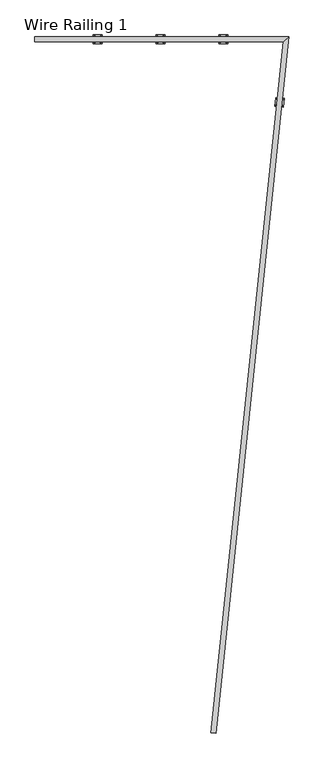
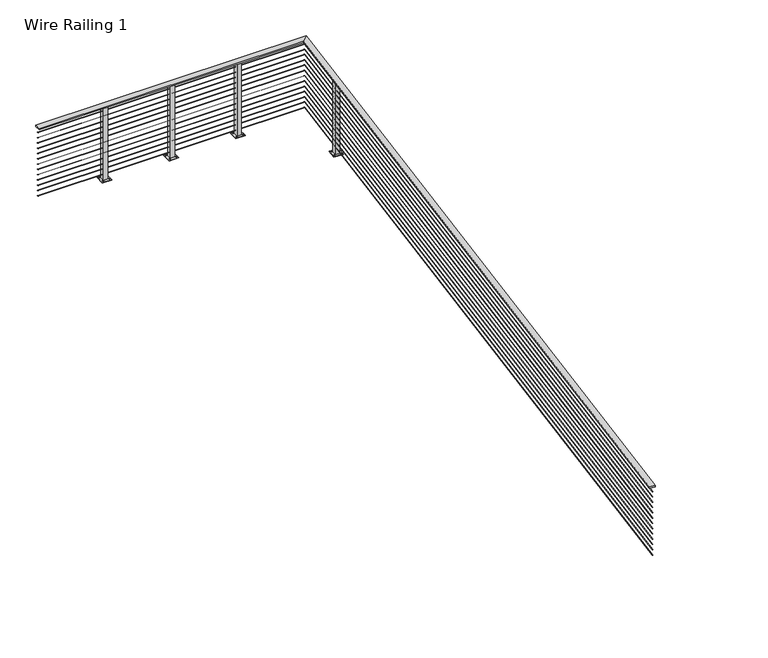
"""IFC4 building model written with IfcOpenShell, lengths in millimetres: railing geometry, Wire Railing 1."""

from ifc_helpers import new_model, si_unit, point, frame, frame_2d, origin, place, context, project, spatial, polyline, circle_curve, ellipse_curve, trimmed, segment, composite_curve, outline, extrude, faceted_brep, source, transform, mapped, element, save
from ifc_brep_helpers import plane_surface, cylinder_surface, advanced_brep


def wire_railing_1_df395d71(model_context):
    return source(origin(), model_context, "Body", "SolidModel", [
        faceted_brep([(31684.2784681, 40829.2481612, 270319.5), (31684.2784681, 40905.4481612, 270319.5), (31684.2784681, 40905.4481612, 270300.45), (31684.2784681, 40829.2481612, 270300.45), (35285.6983833, 40829.2481612, 270300.45), (35285.6983833, 40829.2481612, 270319.5), (35370.327057, 40905.4481612, 270300.45), (35370.327057, 40905.4481612, 270319.5), (34234.7001024, 30829.6674754, 270319.5), (34234.7001024, 30829.6674754, 270300.45), (34310.4826708, 30821.7024065, 270300.45), (34310.4826708, 30821.7024065, 270319.5)], [[[0, 1, 2, 3]], [[4, 5, 0, 3]], [[6, 4, 3, 2]], [[7, 6, 2, 1]], [[5, 7, 1, 0]], [[8, 9, 10, 11]], [[9, 8, 5, 4]], [[10, 9, 4, 6]], [[11, 10, 6, 7]], [[8, 11, 7, 5]]]),
        advanced_brep(
        [(31684.2784681, 40869.7294112, 270240.91875), (31684.2784681, 40864.9669112, 270240.91875), (35325.3680741, 40864.9669112, 270240.91875), (35330.6573662, 40869.7294112, 270240.91875), (34274.9595918, 30825.4360325, 270240.91875), (34270.2231813, 30825.9338493, 270240.91875)],
        [
            (0, 1, circle_curve(frame((31684.2784681, 40867.3481612, 270240.91875), z_axis=(-1.0, 0.0, 0.0), x_axis=(0.0, -1.0, 0.0)), 2.38125)),
            (1, 0, circle_curve(frame((31684.2784681, 40867.3481612, 270240.91875), z_axis=(-1.0, 0.0, 0.0), x_axis=(0.0, -1.0, 0.0)), 2.38125)),
            (2, 3, ellipse_curve(frame((35328.0127201, 40867.3481612, 270240.91875), z_axis=(-0.669130606358848, 0.7431448254774035, 0.0), x_axis=(0.7431448254774035, 0.6691306063588481, 0.0)), 3.5587223, 2.38125)),
            (3, 0),
            (1, 2),
            (3, 2, ellipse_curve(frame((35328.0127201, 40867.3481612, 270240.91875), z_axis=(-0.669130606358848, 0.7431448254774035, 0.0), x_axis=(0.7431448254774035, 0.6691306063588481, 0.0)), 3.5587223, 2.38125)),
            (4, 5, circle_curve(frame((34272.5913866, 30825.6849409, 270240.91875), z_axis=(-0.10452846326767264, -0.9945218953682714, 0.0), x_axis=(-0.9945218953682714, 0.10452846326767264, 0.0)), 2.38125)),
            (5, 4, circle_curve(frame((34272.5913866, 30825.6849409, 270240.91875), z_axis=(-0.10452846326767264, -0.9945218953682714, 0.0), x_axis=(-0.9945218953682714, 0.10452846326767264, 0.0)), 2.38125)),
            (4, 3),
            (2, 5),
        ],
        [
            plane_surface(frame((31684.2784681, 40867.3481612, 270243.3), z_axis=(-1.0, 0.0, 0.0), x_axis=(0.0, -1.0, 0.0))),
            cylinder_surface(frame((35328.0127201, 40867.3481612, 270240.91875), z_axis=(1.0, 0.0, 0.0), x_axis=(0.0, -1.0, 0.0)), 2.38125),
            plane_surface(frame((34272.5913866, 30825.6849409, 270243.3), z_axis=(-0.10452846326767265, -0.9945218953682714, 0.0), x_axis=(0.9945218953682714, -0.10452846326767265, 0.0))),
            cylinder_surface(frame((34272.5913866, 30825.6849409, 270240.91875), z_axis=(-0.10452846326767264, -0.9945218953682714, 0.0), x_axis=(-0.9945218953682714, 0.10452846326767264, 0.0)), 2.38125),
        ],
        [
            (0, [[1, 2]]),
            (1, [[3, 4, -2, 5]]),
            (1, [[6, -5, -1, -4]]),
            (2, [[7, 8]]),
            (3, [[-7, 9, -3, 10]]),
            (3, [[-8, -10, -6, -9]]),
        ],
    ),
        advanced_brep(
        [(31684.2784681, 40869.7294112, 270164.71875), (31684.2784681, 40864.9669112, 270164.71875), (35325.3680741, 40864.9669112, 270164.71875), (35330.6573662, 40869.7294112, 270164.71875), (34274.9595918, 30825.4360325, 270164.71875), (34270.2231813, 30825.9338493, 270164.71875)],
        [
            (0, 1, circle_curve(frame((31684.2784681, 40867.3481612, 270164.71875), z_axis=(-1.0, 0.0, 0.0), x_axis=(0.0, -1.0, 0.0)), 2.38125)),
            (1, 0, circle_curve(frame((31684.2784681, 40867.3481612, 270164.71875), z_axis=(-1.0, 0.0, 0.0), x_axis=(0.0, -1.0, 0.0)), 2.38125)),
            (2, 3, ellipse_curve(frame((35328.0127201, 40867.3481612, 270164.71875), z_axis=(-0.669130606358848, 0.7431448254774035, 0.0), x_axis=(0.7431448254774035, 0.6691306063588481, 0.0)), 3.5587223, 2.38125)),
            (3, 0),
            (1, 2),
            (3, 2, ellipse_curve(frame((35328.0127201, 40867.3481612, 270164.71875), z_axis=(-0.669130606358848, 0.7431448254774035, 0.0), x_axis=(0.7431448254774035, 0.6691306063588481, 0.0)), 3.5587223, 2.38125)),
            (4, 5, circle_curve(frame((34272.5913866, 30825.6849409, 270164.71875), z_axis=(-0.10452846326767264, -0.9945218953682714, 0.0), x_axis=(-0.9945218953682714, 0.10452846326767264, 0.0)), 2.38125)),
            (5, 4, circle_curve(frame((34272.5913866, 30825.6849409, 270164.71875), z_axis=(-0.10452846326767264, -0.9945218953682714, 0.0), x_axis=(-0.9945218953682714, 0.10452846326767264, 0.0)), 2.38125)),
            (4, 3),
            (2, 5),
        ],
        [
            plane_surface(frame((31684.2784681, 40867.3481612, 270167.1), z_axis=(-1.0, 0.0, 0.0), x_axis=(0.0, -1.0, 0.0))),
            cylinder_surface(frame((35328.0127201, 40867.3481612, 270164.71875), z_axis=(1.0, 0.0, 0.0), x_axis=(0.0, -1.0, 0.0)), 2.38125),
            plane_surface(frame((34272.5913866, 30825.6849409, 270167.1), z_axis=(-0.10452846326767265, -0.9945218953682714, 0.0), x_axis=(0.9945218953682714, -0.10452846326767265, 0.0))),
            cylinder_surface(frame((34272.5913866, 30825.6849409, 270164.71875), z_axis=(-0.10452846326767264, -0.9945218953682714, 0.0), x_axis=(-0.9945218953682714, 0.10452846326767264, 0.0)), 2.38125),
        ],
        [
            (0, [[1, 2]]),
            (1, [[3, 4, -2, 5]]),
            (1, [[6, -5, -1, -4]]),
            (2, [[7, 8]]),
            (3, [[-7, 9, -3, 10]]),
            (3, [[-8, -10, -6, -9]]),
        ],
    ),
        advanced_brep(
        [(31684.2784681, 40869.7294112, 270088.51875), (31684.2784681, 40864.9669112, 270088.51875), (35325.3680741, 40864.9669112, 270088.51875), (35330.6573662, 40869.7294112, 270088.51875), (34274.9595918, 30825.4360325, 270088.51875), (34270.2231813, 30825.9338493, 270088.51875)],
        [
            (0, 1, circle_curve(frame((31684.2784681, 40867.3481612, 270088.51875), z_axis=(-1.0, 0.0, 0.0), x_axis=(0.0, -1.0, 0.0)), 2.38125)),
            (1, 0, circle_curve(frame((31684.2784681, 40867.3481612, 270088.51875), z_axis=(-1.0, 0.0, 0.0), x_axis=(0.0, -1.0, 0.0)), 2.38125)),
            (2, 3, ellipse_curve(frame((35328.0127201, 40867.3481612, 270088.51875), z_axis=(-0.669130606358848, 0.7431448254774035, 0.0), x_axis=(0.7431448254774035, 0.6691306063588481, 0.0)), 3.5587223, 2.38125)),
            (3, 0),
            (1, 2),
            (3, 2, ellipse_curve(frame((35328.0127201, 40867.3481612, 270088.51875), z_axis=(-0.669130606358848, 0.7431448254774035, 0.0), x_axis=(0.7431448254774035, 0.6691306063588481, 0.0)), 3.5587223, 2.38125)),
            (4, 5, circle_curve(frame((34272.5913866, 30825.6849409, 270088.51875), z_axis=(-0.10452846326767264, -0.9945218953682714, 0.0), x_axis=(-0.9945218953682714, 0.10452846326767264, 0.0)), 2.38125)),
            (5, 4, circle_curve(frame((34272.5913866, 30825.6849409, 270088.51875), z_axis=(-0.10452846326767264, -0.9945218953682714, 0.0), x_axis=(-0.9945218953682714, 0.10452846326767264, 0.0)), 2.38125)),
            (4, 3),
            (2, 5),
        ],
        [
            plane_surface(frame((31684.2784681, 40867.3481612, 270090.9), z_axis=(-1.0, 0.0, 0.0), x_axis=(0.0, -1.0, 0.0))),
            cylinder_surface(frame((35328.0127201, 40867.3481612, 270088.51875), z_axis=(1.0, 0.0, 0.0), x_axis=(0.0, -1.0, 0.0)), 2.38125),
            plane_surface(frame((34272.5913866, 30825.6849409, 270090.9), z_axis=(-0.10452846326767265, -0.9945218953682714, 0.0), x_axis=(0.9945218953682714, -0.10452846326767265, 0.0))),
            cylinder_surface(frame((34272.5913866, 30825.6849409, 270088.51875), z_axis=(-0.10452846326767264, -0.9945218953682714, 0.0), x_axis=(-0.9945218953682714, 0.10452846326767264, 0.0)), 2.38125),
        ],
        [
            (0, [[1, 2]]),
            (1, [[3, 4, -2, 5]]),
            (1, [[6, -5, -1, -4]]),
            (2, [[7, 8]]),
            (3, [[-7, 9, -3, 10]]),
            (3, [[-8, -10, -6, -9]]),
        ],
    ),
        advanced_brep(
        [(31684.2784681, 40869.7294112, 270012.31875), (31684.2784681, 40864.9669112, 270012.31875), (35325.3680741, 40864.9669112, 270012.31875), (35330.6573662, 40869.7294112, 270012.31875), (34274.9595918, 30825.4360325, 270012.31875), (34270.2231813, 30825.9338493, 270012.31875)],
        [
            (0, 1, circle_curve(frame((31684.2784681, 40867.3481612, 270012.31875), z_axis=(-1.0, 0.0, 0.0), x_axis=(0.0, -1.0, 0.0)), 2.38125)),
            (1, 0, circle_curve(frame((31684.2784681, 40867.3481612, 270012.31875), z_axis=(-1.0, 0.0, 0.0), x_axis=(0.0, -1.0, 0.0)), 2.38125)),
            (2, 3, ellipse_curve(frame((35328.0127201, 40867.3481612, 270012.31875), z_axis=(-0.669130606358848, 0.7431448254774035, 0.0), x_axis=(0.7431448254774035, 0.6691306063588481, 0.0)), 3.5587223, 2.38125)),
            (3, 0),
            (1, 2),
            (3, 2, ellipse_curve(frame((35328.0127201, 40867.3481612, 270012.31875), z_axis=(-0.669130606358848, 0.7431448254774035, 0.0), x_axis=(0.7431448254774035, 0.6691306063588481, 0.0)), 3.5587223, 2.38125)),
            (4, 5, circle_curve(frame((34272.5913866, 30825.6849409, 270012.31875), z_axis=(-0.10452846326767264, -0.9945218953682714, 0.0), x_axis=(-0.9945218953682714, 0.10452846326767264, 0.0)), 2.38125)),
            (5, 4, circle_curve(frame((34272.5913866, 30825.6849409, 270012.31875), z_axis=(-0.10452846326767264, -0.9945218953682714, 0.0), x_axis=(-0.9945218953682714, 0.10452846326767264, 0.0)), 2.38125)),
            (4, 3),
            (2, 5),
        ],
        [
            plane_surface(frame((31684.2784681, 40867.3481612, 270014.7), z_axis=(-1.0, 0.0, 0.0), x_axis=(0.0, -1.0, 0.0))),
            cylinder_surface(frame((35328.0127201, 40867.3481612, 270012.31875), z_axis=(1.0, 0.0, 0.0), x_axis=(0.0, -1.0, 0.0)), 2.38125),
            plane_surface(frame((34272.5913866, 30825.6849409, 270014.7), z_axis=(-0.10452846326767265, -0.9945218953682714, 0.0), x_axis=(0.9945218953682714, -0.10452846326767265, 0.0))),
            cylinder_surface(frame((34272.5913866, 30825.6849409, 270012.31875), z_axis=(-0.10452846326767264, -0.9945218953682714, 0.0), x_axis=(-0.9945218953682714, 0.10452846326767264, 0.0)), 2.38125),
        ],
        [
            (0, [[1, 2]]),
            (1, [[3, 4, -2, 5]]),
            (1, [[6, -5, -1, -4]]),
            (2, [[7, 8]]),
            (3, [[-7, 9, -3, 10]]),
            (3, [[-8, -10, -6, -9]]),
        ],
    ),
        advanced_brep(
        [(31684.2784681, 40869.7294112, 269936.11875), (31684.2784681, 40864.9669112, 269936.11875), (35325.3680741, 40864.9669112, 269936.11875), (35330.6573662, 40869.7294112, 269936.11875), (34274.9595918, 30825.4360325, 269936.11875), (34270.2231813, 30825.9338493, 269936.11875)],
        [
            (0, 1, circle_curve(frame((31684.2784681, 40867.3481612, 269936.11875), z_axis=(-1.0, 0.0, 0.0), x_axis=(0.0, -1.0, 0.0)), 2.38125)),
            (1, 0, circle_curve(frame((31684.2784681, 40867.3481612, 269936.11875), z_axis=(-1.0, 0.0, 0.0), x_axis=(0.0, -1.0, 0.0)), 2.38125)),
            (2, 3, ellipse_curve(frame((35328.0127201, 40867.3481612, 269936.11875), z_axis=(-0.669130606358848, 0.7431448254774035, 0.0), x_axis=(0.7431448254774035, 0.6691306063588481, 0.0)), 3.5587223, 2.38125)),
            (3, 0),
            (1, 2),
            (3, 2, ellipse_curve(frame((35328.0127201, 40867.3481612, 269936.11875), z_axis=(-0.669130606358848, 0.7431448254774035, 0.0), x_axis=(0.7431448254774035, 0.6691306063588481, 0.0)), 3.5587223, 2.38125)),
            (4, 5, circle_curve(frame((34272.5913866, 30825.6849409, 269936.11875), z_axis=(-0.10452846326767264, -0.9945218953682714, 0.0), x_axis=(-0.9945218953682714, 0.10452846326767264, 0.0)), 2.38125)),
            (5, 4, circle_curve(frame((34272.5913866, 30825.6849409, 269936.11875), z_axis=(-0.10452846326767264, -0.9945218953682714, 0.0), x_axis=(-0.9945218953682714, 0.10452846326767264, 0.0)), 2.38125)),
            (4, 3),
            (2, 5),
        ],
        [
            plane_surface(frame((31684.2784681, 40867.3481612, 269938.5), z_axis=(-1.0, 0.0, 0.0), x_axis=(0.0, -1.0, 0.0))),
            cylinder_surface(frame((35328.0127201, 40867.3481612, 269936.11875), z_axis=(1.0, 0.0, 0.0), x_axis=(0.0, -1.0, 0.0)), 2.38125),
            plane_surface(frame((34272.5913866, 30825.6849409, 269938.5), z_axis=(-0.10452846326767265, -0.9945218953682714, 0.0), x_axis=(0.9945218953682714, -0.10452846326767265, 0.0))),
            cylinder_surface(frame((34272.5913866, 30825.6849409, 269936.11875), z_axis=(-0.10452846326767264, -0.9945218953682714, 0.0), x_axis=(-0.9945218953682714, 0.10452846326767264, 0.0)), 2.38125),
        ],
        [
            (0, [[1, 2]]),
            (1, [[3, 4, -2, 5]]),
            (1, [[6, -5, -1, -4]]),
            (2, [[7, 8]]),
            (3, [[-7, 9, -3, 10]]),
            (3, [[-8, -10, -6, -9]]),
        ],
    ),
        advanced_brep(
        [(31684.2784681, 40869.7294112, 269859.91875), (31684.2784681, 40864.9669112, 269859.91875), (35325.3680741, 40864.9669112, 269859.91875), (35330.6573662, 40869.7294112, 269859.91875), (34274.9595918, 30825.4360325, 269859.91875), (34270.2231813, 30825.9338493, 269859.91875)],
        [
            (0, 1, circle_curve(frame((31684.2784681, 40867.3481612, 269859.91875), z_axis=(-1.0, 0.0, 0.0), x_axis=(0.0, -1.0, 0.0)), 2.38125)),
            (1, 0, circle_curve(frame((31684.2784681, 40867.3481612, 269859.91875), z_axis=(-1.0, 0.0, 0.0), x_axis=(0.0, -1.0, 0.0)), 2.38125)),
            (2, 3, ellipse_curve(frame((35328.0127201, 40867.3481612, 269859.91875), z_axis=(-0.669130606358848, 0.7431448254774035, 0.0), x_axis=(0.7431448254774035, 0.6691306063588481, 0.0)), 3.5587223, 2.38125)),
            (3, 0),
            (1, 2),
            (3, 2, ellipse_curve(frame((35328.0127201, 40867.3481612, 269859.91875), z_axis=(-0.669130606358848, 0.7431448254774035, 0.0), x_axis=(0.7431448254774035, 0.6691306063588481, 0.0)), 3.5587223, 2.38125)),
            (4, 5, circle_curve(frame((34272.5913866, 30825.6849409, 269859.91875), z_axis=(-0.10452846326767264, -0.9945218953682714, 0.0), x_axis=(-0.9945218953682714, 0.10452846326767264, 0.0)), 2.38125)),
            (5, 4, circle_curve(frame((34272.5913866, 30825.6849409, 269859.91875), z_axis=(-0.10452846326767264, -0.9945218953682714, 0.0), x_axis=(-0.9945218953682714, 0.10452846326767264, 0.0)), 2.38125)),
            (4, 3),
            (2, 5),
        ],
        [
            plane_surface(frame((31684.2784681, 40867.3481612, 269862.3), z_axis=(-1.0, 0.0, 0.0), x_axis=(0.0, -1.0, 0.0))),
            cylinder_surface(frame((35328.0127201, 40867.3481612, 269859.91875), z_axis=(1.0, 0.0, 0.0), x_axis=(0.0, -1.0, 0.0)), 2.38125),
            plane_surface(frame((34272.5913866, 30825.6849409, 269862.3), z_axis=(-0.10452846326767265, -0.9945218953682714, 0.0), x_axis=(0.9945218953682714, -0.10452846326767265, 0.0))),
            cylinder_surface(frame((34272.5913866, 30825.6849409, 269859.91875), z_axis=(-0.10452846326767264, -0.9945218953682714, 0.0), x_axis=(-0.9945218953682714, 0.10452846326767264, 0.0)), 2.38125),
        ],
        [
            (0, [[1, 2]]),
            (1, [[3, 4, -2, 5]]),
            (1, [[6, -5, -1, -4]]),
            (2, [[7, 8]]),
            (3, [[-7, 9, -3, 10]]),
            (3, [[-8, -10, -6, -9]]),
        ],
    ),
        advanced_brep(
        [(31684.2784681, 40869.7294112, 269783.71875), (31684.2784681, 40864.9669112, 269783.71875), (35325.3680741, 40864.9669112, 269783.71875), (35330.6573662, 40869.7294112, 269783.71875), (34274.9595918, 30825.4360325, 269783.71875), (34270.2231813, 30825.9338493, 269783.71875)],
        [
            (0, 1, circle_curve(frame((31684.2784681, 40867.3481612, 269783.71875), z_axis=(-1.0, 0.0, 0.0), x_axis=(0.0, -1.0, 0.0)), 2.38125)),
            (1, 0, circle_curve(frame((31684.2784681, 40867.3481612, 269783.71875), z_axis=(-1.0, 0.0, 0.0), x_axis=(0.0, -1.0, 0.0)), 2.38125)),
            (2, 3, ellipse_curve(frame((35328.0127201, 40867.3481612, 269783.71875), z_axis=(-0.669130606358848, 0.7431448254774035, 0.0), x_axis=(0.7431448254774035, 0.6691306063588481, 0.0)), 3.5587223, 2.38125)),
            (3, 0),
            (1, 2),
            (3, 2, ellipse_curve(frame((35328.0127201, 40867.3481612, 269783.71875), z_axis=(-0.669130606358848, 0.7431448254774035, 0.0), x_axis=(0.7431448254774035, 0.6691306063588481, 0.0)), 3.5587223, 2.38125)),
            (4, 5, circle_curve(frame((34272.5913866, 30825.6849409, 269783.71875), z_axis=(-0.10452846326767264, -0.9945218953682714, 0.0), x_axis=(-0.9945218953682714, 0.10452846326767264, 0.0)), 2.38125)),
            (5, 4, circle_curve(frame((34272.5913866, 30825.6849409, 269783.71875), z_axis=(-0.10452846326767264, -0.9945218953682714, 0.0), x_axis=(-0.9945218953682714, 0.10452846326767264, 0.0)), 2.38125)),
            (4, 3),
            (2, 5),
        ],
        [
            plane_surface(frame((31684.2784681, 40867.3481612, 269786.1), z_axis=(-1.0, 0.0, 0.0), x_axis=(0.0, -1.0, 0.0))),
            cylinder_surface(frame((35328.0127201, 40867.3481612, 269783.71875), z_axis=(1.0, 0.0, 0.0), x_axis=(0.0, -1.0, 0.0)), 2.38125),
            plane_surface(frame((34272.5913866, 30825.6849409, 269786.1), z_axis=(-0.10452846326767265, -0.9945218953682714, 0.0), x_axis=(0.9945218953682714, -0.10452846326767265, 0.0))),
            cylinder_surface(frame((34272.5913866, 30825.6849409, 269783.71875), z_axis=(-0.10452846326767264, -0.9945218953682714, 0.0), x_axis=(-0.9945218953682714, 0.10452846326767264, 0.0)), 2.38125),
        ],
        [
            (0, [[1, 2]]),
            (1, [[3, 4, -2, 5]]),
            (1, [[6, -5, -1, -4]]),
            (2, [[7, 8]]),
            (3, [[-7, 9, -3, 10]]),
            (3, [[-8, -10, -6, -9]]),
        ],
    ),
        advanced_brep(
        [(31684.2784681, 40869.7294112, 269707.51875), (31684.2784681, 40864.9669112, 269707.51875), (35325.3680741, 40864.9669112, 269707.51875), (35330.6573662, 40869.7294112, 269707.51875), (34274.9595918, 30825.4360325, 269707.51875), (34270.2231813, 30825.9338493, 269707.51875)],
        [
            (0, 1, circle_curve(frame((31684.2784681, 40867.3481612, 269707.51875), z_axis=(-1.0, 0.0, 0.0), x_axis=(0.0, -1.0, 0.0)), 2.38125)),
            (1, 0, circle_curve(frame((31684.2784681, 40867.3481612, 269707.51875), z_axis=(-1.0, 0.0, 0.0), x_axis=(0.0, -1.0, 0.0)), 2.38125)),
            (2, 3, ellipse_curve(frame((35328.0127201, 40867.3481612, 269707.51875), z_axis=(-0.669130606358848, 0.7431448254774035, 0.0), x_axis=(0.7431448254774035, 0.6691306063588481, 0.0)), 3.5587223, 2.38125)),
            (3, 0),
            (1, 2),
            (3, 2, ellipse_curve(frame((35328.0127201, 40867.3481612, 269707.51875), z_axis=(-0.669130606358848, 0.7431448254774035, 0.0), x_axis=(0.7431448254774035, 0.6691306063588481, 0.0)), 3.5587223, 2.38125)),
            (4, 5, circle_curve(frame((34272.5913866, 30825.6849409, 269707.51875), z_axis=(-0.10452846326767264, -0.9945218953682714, 0.0), x_axis=(-0.9945218953682714, 0.10452846326767264, 0.0)), 2.38125)),
            (5, 4, circle_curve(frame((34272.5913866, 30825.6849409, 269707.51875), z_axis=(-0.10452846326767264, -0.9945218953682714, 0.0), x_axis=(-0.9945218953682714, 0.10452846326767264, 0.0)), 2.38125)),
            (4, 3),
            (2, 5),
        ],
        [
            plane_surface(frame((31684.2784681, 40867.3481612, 269709.9), z_axis=(-1.0, 0.0, 0.0), x_axis=(0.0, -1.0, 0.0))),
            cylinder_surface(frame((35328.0127201, 40867.3481612, 269707.51875), z_axis=(1.0, 0.0, 0.0), x_axis=(0.0, -1.0, 0.0)), 2.38125),
            plane_surface(frame((34272.5913866, 30825.6849409, 269709.9), z_axis=(-0.10452846326767265, -0.9945218953682714, 0.0), x_axis=(0.9945218953682714, -0.10452846326767265, 0.0))),
            cylinder_surface(frame((34272.5913866, 30825.6849409, 269707.51875), z_axis=(-0.10452846326767264, -0.9945218953682714, 0.0), x_axis=(-0.9945218953682714, 0.10452846326767264, 0.0)), 2.38125),
        ],
        [
            (0, [[1, 2]]),
            (1, [[3, 4, -2, 5]]),
            (1, [[6, -5, -1, -4]]),
            (2, [[7, 8]]),
            (3, [[-7, 9, -3, 10]]),
            (3, [[-8, -10, -6, -9]]),
        ],
    ),
        advanced_brep(
        [(31684.2784681, 40869.7294112, 269631.31875), (31684.2784681, 40864.9669112, 269631.31875), (35325.3680741, 40864.9669112, 269631.31875), (35330.6573662, 40869.7294112, 269631.31875), (34274.9595918, 30825.4360325, 269631.31875), (34270.2231813, 30825.9338493, 269631.31875)],
        [
            (0, 1, circle_curve(frame((31684.2784681, 40867.3481612, 269631.31875), z_axis=(-1.0, 0.0, 0.0), x_axis=(0.0, -1.0, 0.0)), 2.38125)),
            (1, 0, circle_curve(frame((31684.2784681, 40867.3481612, 269631.31875), z_axis=(-1.0, 0.0, 0.0), x_axis=(0.0, -1.0, 0.0)), 2.38125)),
            (2, 3, ellipse_curve(frame((35328.0127201, 40867.3481612, 269631.31875), z_axis=(-0.669130606358848, 0.7431448254774035, 0.0), x_axis=(0.7431448254774035, 0.6691306063588481, 0.0)), 3.5587223, 2.38125)),
            (3, 0),
            (1, 2),
            (3, 2, ellipse_curve(frame((35328.0127201, 40867.3481612, 269631.31875), z_axis=(-0.669130606358848, 0.7431448254774035, 0.0), x_axis=(0.7431448254774035, 0.6691306063588481, 0.0)), 3.5587223, 2.38125)),
            (4, 5, circle_curve(frame((34272.5913866, 30825.6849409, 269631.31875), z_axis=(-0.10452846326767264, -0.9945218953682714, 0.0), x_axis=(-0.9945218953682714, 0.10452846326767264, 0.0)), 2.38125)),
            (5, 4, circle_curve(frame((34272.5913866, 30825.6849409, 269631.31875), z_axis=(-0.10452846326767264, -0.9945218953682714, 0.0), x_axis=(-0.9945218953682714, 0.10452846326767264, 0.0)), 2.38125)),
            (4, 3),
            (2, 5),
        ],
        [
            plane_surface(frame((31684.2784681, 40867.3481612, 269633.7), z_axis=(-1.0, 0.0, 0.0), x_axis=(0.0, -1.0, 0.0))),
            cylinder_surface(frame((35328.0127201, 40867.3481612, 269631.31875), z_axis=(1.0, 0.0, 0.0), x_axis=(0.0, -1.0, 0.0)), 2.38125),
            plane_surface(frame((34272.5913866, 30825.6849409, 269633.7), z_axis=(-0.10452846326767265, -0.9945218953682714, 0.0), x_axis=(0.9945218953682714, -0.10452846326767265, 0.0))),
            cylinder_surface(frame((34272.5913866, 30825.6849409, 269631.31875), z_axis=(-0.10452846326767264, -0.9945218953682714, 0.0), x_axis=(-0.9945218953682714, 0.10452846326767264, 0.0)), 2.38125),
        ],
        [
            (0, [[1, 2]]),
            (1, [[3, 4, -2, 5]]),
            (1, [[6, -5, -1, -4]]),
            (2, [[7, 8]]),
            (3, [[-7, 9, -3, 10]]),
            (3, [[-8, -10, -6, -9]]),
        ],
    ),
        advanced_brep(
        [(31684.2784681, 40869.7294112, 269555.11875), (31684.2784681, 40864.9669112, 269555.11875), (35325.3680741, 40864.9669112, 269555.11875), (35330.6573662, 40869.7294112, 269555.11875), (34274.9595918, 30825.4360325, 269555.11875), (34270.2231813, 30825.9338493, 269555.11875)],
        [
            (0, 1, circle_curve(frame((31684.2784681, 40867.3481612, 269555.11875), z_axis=(-1.0, 0.0, 0.0), x_axis=(0.0, -1.0, 0.0)), 2.38125)),
            (1, 0, circle_curve(frame((31684.2784681, 40867.3481612, 269555.11875), z_axis=(-1.0, 0.0, 0.0), x_axis=(0.0, -1.0, 0.0)), 2.38125)),
            (2, 3, ellipse_curve(frame((35328.0127201, 40867.3481612, 269555.11875), z_axis=(-0.669130606358848, 0.7431448254774035, 0.0), x_axis=(0.7431448254774035, 0.6691306063588481, 0.0)), 3.5587223, 2.38125)),
            (3, 0),
            (1, 2),
            (3, 2, ellipse_curve(frame((35328.0127201, 40867.3481612, 269555.11875), z_axis=(-0.669130606358848, 0.7431448254774035, 0.0), x_axis=(0.7431448254774035, 0.6691306063588481, 0.0)), 3.5587223, 2.38125)),
            (4, 5, circle_curve(frame((34272.5913866, 30825.6849409, 269555.11875), z_axis=(-0.10452846326767264, -0.9945218953682714, 0.0), x_axis=(-0.9945218953682714, 0.10452846326767264, 0.0)), 2.38125)),
            (5, 4, circle_curve(frame((34272.5913866, 30825.6849409, 269555.11875), z_axis=(-0.10452846326767264, -0.9945218953682714, 0.0), x_axis=(-0.9945218953682714, 0.10452846326767264, 0.0)), 2.38125)),
            (4, 3),
            (2, 5),
        ],
        [
            plane_surface(frame((31684.2784681, 40867.3481612, 269557.5), z_axis=(-1.0, 0.0, 0.0), x_axis=(0.0, -1.0, 0.0))),
            cylinder_surface(frame((35328.0127201, 40867.3481612, 269555.11875), z_axis=(1.0, 0.0, 0.0), x_axis=(0.0, -1.0, 0.0)), 2.38125),
            plane_surface(frame((34272.5913866, 30825.6849409, 269557.5), z_axis=(-0.10452846326767265, -0.9945218953682714, 0.0), x_axis=(0.9945218953682714, -0.10452846326767265, 0.0))),
            cylinder_surface(frame((34272.5913866, 30825.6849409, 269555.11875), z_axis=(-0.10452846326767264, -0.9945218953682714, 0.0), x_axis=(-0.9945218953682714, 0.10452846326767264, 0.0)), 2.38125),
        ],
        [
            (0, [[1, 2]]),
            (1, [[3, 4, -2, 5]]),
            (1, [[6, -5, -1, -4]]),
            (2, [[7, 8]]),
            (3, [[-7, 9, -3, 10]]),
            (3, [[-8, -10, -6, -9]]),
        ],
    ),
        advanced_brep(
        [(31684.2784681, 40869.7294112, 269478.91875), (31684.2784681, 40864.9669112, 269478.91875), (35325.3680741, 40864.9669112, 269478.91875), (35330.6573662, 40869.7294112, 269478.91875), (34274.9595918, 30825.4360325, 269478.91875), (34270.2231813, 30825.9338493, 269478.91875)],
        [
            (0, 1, circle_curve(frame((31684.2784681, 40867.3481612, 269478.91875), z_axis=(-1.0, 0.0, 0.0), x_axis=(0.0, -1.0, 0.0)), 2.38125)),
            (1, 0, circle_curve(frame((31684.2784681, 40867.3481612, 269478.91875), z_axis=(-1.0, 0.0, 0.0), x_axis=(0.0, -1.0, 0.0)), 2.38125)),
            (2, 3, ellipse_curve(frame((35328.0127201, 40867.3481612, 269478.91875), z_axis=(-0.669130606358848, 0.7431448254774035, 0.0), x_axis=(0.7431448254774035, 0.6691306063588481, 0.0)), 3.5587223, 2.38125)),
            (3, 0),
            (1, 2),
            (3, 2, ellipse_curve(frame((35328.0127201, 40867.3481612, 269478.91875), z_axis=(-0.669130606358848, 0.7431448254774035, 0.0), x_axis=(0.7431448254774035, 0.6691306063588481, 0.0)), 3.5587223, 2.38125)),
            (4, 5, circle_curve(frame((34272.5913866, 30825.6849409, 269478.91875), z_axis=(-0.10452846326767264, -0.9945218953682714, 0.0), x_axis=(-0.9945218953682714, 0.10452846326767264, 0.0)), 2.38125)),
            (5, 4, circle_curve(frame((34272.5913866, 30825.6849409, 269478.91875), z_axis=(-0.10452846326767264, -0.9945218953682714, 0.0), x_axis=(-0.9945218953682714, 0.10452846326767264, 0.0)), 2.38125)),
            (4, 3),
            (2, 5),
        ],
        [
            plane_surface(frame((31684.2784681, 40867.3481612, 269481.3), z_axis=(-1.0, 0.0, 0.0), x_axis=(0.0, -1.0, 0.0))),
            cylinder_surface(frame((35328.0127201, 40867.3481612, 269478.91875), z_axis=(1.0, 0.0, 0.0), x_axis=(0.0, -1.0, 0.0)), 2.38125),
            plane_surface(frame((34272.5913866, 30825.6849409, 269481.3), z_axis=(-0.10452846326767265, -0.9945218953682714, 0.0), x_axis=(0.9945218953682714, -0.10452846326767265, 0.0))),
            cylinder_surface(frame((34272.5913866, 30825.6849409, 269478.91875), z_axis=(-0.10452846326767264, -0.9945218953682714, 0.0), x_axis=(-0.9945218953682714, 0.10452846326767264, 0.0)), 2.38125),
        ],
        [
            (0, [[1, 2]]),
            (1, [[3, 4, -2, 5]]),
            (1, [[6, -5, -1, -4]]),
            (2, [[7, 8]]),
            (3, [[-7, 9, -3, 10]]),
            (3, [[-8, -10, -6, -9]]),
        ],
    ),
        advanced_brep(
        [(31684.2784681, 40869.7294112, 269402.71875), (31684.2784681, 40864.9669112, 269402.71875), (35325.3680741, 40864.9669112, 269402.71875), (35330.6573662, 40869.7294112, 269402.71875), (34274.9595918, 30825.4360325, 269402.71875), (34270.2231813, 30825.9338493, 269402.71875)],
        [
            (0, 1, circle_curve(frame((31684.2784681, 40867.3481612, 269402.71875), z_axis=(-1.0, 0.0, 0.0), x_axis=(0.0, -1.0, 0.0)), 2.38125)),
            (1, 0, circle_curve(frame((31684.2784681, 40867.3481612, 269402.71875), z_axis=(-1.0, 0.0, 0.0), x_axis=(0.0, -1.0, 0.0)), 2.38125)),
            (2, 3, ellipse_curve(frame((35328.0127201, 40867.3481612, 269402.71875), z_axis=(-0.669130606358848, 0.7431448254774035, 0.0), x_axis=(0.7431448254774035, 0.6691306063588481, 0.0)), 3.5587223, 2.38125)),
            (3, 0),
            (1, 2),
            (3, 2, ellipse_curve(frame((35328.0127201, 40867.3481612, 269402.71875), z_axis=(-0.669130606358848, 0.7431448254774035, 0.0), x_axis=(0.7431448254774035, 0.6691306063588481, 0.0)), 3.5587223, 2.38125)),
            (4, 5, circle_curve(frame((34272.5913866, 30825.6849409, 269402.71875), z_axis=(-0.10452846326767264, -0.9945218953682714, 0.0), x_axis=(-0.9945218953682714, 0.10452846326767264, 0.0)), 2.38125)),
            (5, 4, circle_curve(frame((34272.5913866, 30825.6849409, 269402.71875), z_axis=(-0.10452846326767264, -0.9945218953682714, 0.0), x_axis=(-0.9945218953682714, 0.10452846326767264, 0.0)), 2.38125)),
            (4, 3),
            (2, 5),
        ],
        [
            plane_surface(frame((31684.2784681, 40867.3481612, 269405.1), z_axis=(-1.0, 0.0, 0.0), x_axis=(0.0, -1.0, 0.0))),
            cylinder_surface(frame((35328.0127201, 40867.3481612, 269402.71875), z_axis=(1.0, 0.0, 0.0), x_axis=(0.0, -1.0, 0.0)), 2.38125),
            plane_surface(frame((34272.5913866, 30825.6849409, 269405.1), z_axis=(-0.10452846326767265, -0.9945218953682714, 0.0), x_axis=(0.9945218953682714, -0.10452846326767265, 0.0))),
            cylinder_surface(frame((34272.5913866, 30825.6849409, 269402.71875), z_axis=(-0.10452846326767264, -0.9945218953682714, 0.0), x_axis=(-0.9945218953682714, 0.10452846326767264, 0.0)), 2.38125),
        ],
        [
            (0, [[1, 2]]),
            (1, [[3, 4, -2, 5]]),
            (1, [[6, -5, -1, -4]]),
            (2, [[7, 8]]),
            (3, [[-7, 9, -3, 10]]),
            (3, [[-8, -10, -6, -9]]),
        ],
    ),
        advanced_brep(
        [(31684.2784681, 40869.7294112, 269326.51875), (31684.2784681, 40864.9669112, 269326.51875), (35325.3680741, 40864.9669112, 269326.51875), (35330.6573662, 40869.7294112, 269326.51875), (34274.9595918, 30825.4360325, 269326.51875), (34270.2231813, 30825.9338493, 269326.51875)],
        [
            (0, 1, circle_curve(frame((31684.2784681, 40867.3481612, 269326.51875), z_axis=(-1.0, 0.0, 0.0), x_axis=(0.0, -1.0, 0.0)), 2.38125)),
            (1, 0, circle_curve(frame((31684.2784681, 40867.3481612, 269326.51875), z_axis=(-1.0, 0.0, 0.0), x_axis=(0.0, -1.0, 0.0)), 2.38125)),
            (2, 3, ellipse_curve(frame((35328.0127201, 40867.3481612, 269326.51875), z_axis=(-0.669130606358848, 0.7431448254774035, 0.0), x_axis=(0.7431448254774035, 0.6691306063588481, 0.0)), 3.5587223, 2.38125)),
            (3, 0),
            (1, 2),
            (3, 2, ellipse_curve(frame((35328.0127201, 40867.3481612, 269326.51875), z_axis=(-0.669130606358848, 0.7431448254774035, 0.0), x_axis=(0.7431448254774035, 0.6691306063588481, 0.0)), 3.5587223, 2.38125)),
            (4, 5, circle_curve(frame((34272.5913866, 30825.6849409, 269326.51875), z_axis=(-0.10452846326767264, -0.9945218953682714, 0.0), x_axis=(-0.9945218953682714, 0.10452846326767264, 0.0)), 2.38125)),
            (5, 4, circle_curve(frame((34272.5913866, 30825.6849409, 269326.51875), z_axis=(-0.10452846326767264, -0.9945218953682714, 0.0), x_axis=(-0.9945218953682714, 0.10452846326767264, 0.0)), 2.38125)),
            (4, 3),
            (2, 5),
        ],
        [
            plane_surface(frame((31684.2784681, 40867.3481612, 269328.9), z_axis=(-1.0, 0.0, 0.0), x_axis=(0.0, -1.0, 0.0))),
            cylinder_surface(frame((35328.0127201, 40867.3481612, 269326.51875), z_axis=(1.0, 0.0, 0.0), x_axis=(0.0, -1.0, 0.0)), 2.38125),
            plane_surface(frame((34272.5913866, 30825.6849409, 269328.9), z_axis=(-0.10452846326767265, -0.9945218953682714, 0.0), x_axis=(0.9945218953682714, -0.10452846326767265, 0.0))),
            cylinder_surface(frame((34272.5913866, 30825.6849409, 269326.51875), z_axis=(-0.10452846326767264, -0.9945218953682714, 0.0), x_axis=(-0.9945218953682714, 0.10452846326767264, 0.0)), 2.38125),
        ],
        [
            (0, [[1, 2]]),
            (1, [[3, 4, -2, 5]]),
            (1, [[6, -5, -1, -4]]),
            (2, [[7, 8]]),
            (3, [[-7, 9, -3, 10]]),
            (3, [[-8, -10, -6, -9]]),
        ],
    ),
        extrude(outline(composite_curve([segment(trimmed(circle_curve(frame_2d((32639.6620311, 40822.8981612)), 6.35), [point((32639.6620311, 40816.5481612))], [point((32639.6620311, 40829.2481612))], False, "CARTESIAN"), True, "CONTINUOUS"), segment(trimmed(circle_curve(frame_2d((32639.6620311, 40822.8981612)), 6.35), [point((32639.6620311, 40829.2481612))], [point((32639.6620311, 40816.5481612))], False, "CARTESIAN"), True, "CONTINUOUS")], self_intersect=False)), frame((0.0, 0.0, 269252.7), z_axis=(0.0, 0.0, 1.0), x_axis=(1.0, 0.0, 0.0)), (0.0, 0.0, 1.0), 12.7),
        extrude(outline(composite_curve([segment(trimmed(circle_curve(frame_2d((32639.6620311, 40911.7981612)), 6.35), [point((32639.6620311, 40905.4481612))], [point((32639.6620311, 40918.1481612))], False, "CARTESIAN"), True, "CONTINUOUS"), segment(trimmed(circle_curve(frame_2d((32639.6620311, 40911.7981612)), 6.35), [point((32639.6620311, 40918.1481612))], [point((32639.6620311, 40905.4481612))], False, "CARTESIAN"), True, "CONTINUOUS")], self_intersect=False)), frame((0.0, 0.0, 269252.7), z_axis=(0.0, 0.0, 1.0), x_axis=(1.0, 0.0, 0.0)), (0.0, 0.0, 1.0), 12.7),
        extrude(outline(composite_curve([segment(trimmed(circle_curve(frame_2d((32550.7620311, 40822.8981612)), 6.35), [point((32550.7620311, 40816.5481612))], [point((32550.7620311, 40829.2481612))], False, "CARTESIAN"), True, "CONTINUOUS"), segment(trimmed(circle_curve(frame_2d((32550.7620311, 40822.8981612)), 6.35), [point((32550.7620311, 40829.2481612))], [point((32550.7620311, 40816.5481612))], False, "CARTESIAN"), True, "CONTINUOUS")], self_intersect=False)), frame((0.0, 0.0, 269252.7), z_axis=(0.0, 0.0, 1.0), x_axis=(1.0, 0.0, 0.0)), (0.0, 0.0, 1.0), 12.7),
        extrude(outline(composite_curve([segment(trimmed(circle_curve(frame_2d((32550.7620311, 40911.7981612)), 6.35), [point((32550.7620311, 40905.4481612))], [point((32550.7620311, 40918.1481612))], False, "CARTESIAN"), True, "CONTINUOUS"), segment(trimmed(circle_curve(frame_2d((32550.7620311, 40911.7981612)), 6.35), [point((32550.7620311, 40918.1481612))], [point((32550.7620311, 40905.4481612))], False, "CARTESIAN"), True, "CONTINUOUS")], self_intersect=False)), frame((0.0, 0.0, 269252.7), z_axis=(0.0, 0.0, 1.0), x_axis=(1.0, 0.0, 0.0)), (0.0, 0.0, 1.0), 12.7),
        extrude(outline(polyline([(32658.7120311, 40930.8481612), (32658.7120311, 40803.8481612), (32531.7120311, 40803.8481612), (32531.7120311, 40930.8481612), (32658.7120311, 40930.8481612)])), frame((0.0, 0.0, 269252.7), z_axis=(0.0, 0.0, 1.0), x_axis=(1.0, 0.0, 0.0)), (0.0, 0.0, 1.0), 6.35),
        extrude(outline(polyline([(32625.3745311, 40897.5106612), (32625.3745311, 40837.1856612), (32565.0495311, 40837.1856612), (32565.0495311, 40897.5106612), (32625.3745311, 40897.5106612)]), holes=[polyline([(32619.0245311, 40891.1606612), (32571.3995311, 40891.1606612), (32571.3995311, 40843.5356612), (32619.0245311, 40843.5356612), (32619.0245311, 40891.1606612)])]), frame((0.0, 0.0, 269252.7), z_axis=(0.0, 0.0, 1.0), x_axis=(1.0, 0.0, 0.0)), (0.0, 0.0, 1.0), 1047.75),
        extrude(outline(composite_curve([segment(trimmed(circle_curve(frame_2d((33550.5955941, 40822.8981612)), 6.35), [point((33550.5955941, 40816.5481612))], [point((33550.5955941, 40829.2481612))], False, "CARTESIAN"), True, "CONTINUOUS"), segment(trimmed(circle_curve(frame_2d((33550.5955941, 40822.8981612)), 6.35), [point((33550.5955941, 40829.2481612))], [point((33550.5955941, 40816.5481612))], False, "CARTESIAN"), True, "CONTINUOUS")], self_intersect=False)), frame((0.0, 0.0, 269252.7), z_axis=(0.0, 0.0, 1.0), x_axis=(1.0, 0.0, 0.0)), (0.0, 0.0, 1.0), 12.7),
        extrude(outline(composite_curve([segment(trimmed(circle_curve(frame_2d((33550.5955941, 40911.7981612)), 6.35), [point((33550.5955941, 40905.4481612))], [point((33550.5955941, 40918.1481612))], False, "CARTESIAN"), True, "CONTINUOUS"), segment(trimmed(circle_curve(frame_2d((33550.5955941, 40911.7981612)), 6.35), [point((33550.5955941, 40918.1481612))], [point((33550.5955941, 40905.4481612))], False, "CARTESIAN"), True, "CONTINUOUS")], self_intersect=False)), frame((0.0, 0.0, 269252.7), z_axis=(0.0, 0.0, 1.0), x_axis=(1.0, 0.0, 0.0)), (0.0, 0.0, 1.0), 12.7),
        extrude(outline(composite_curve([segment(trimmed(circle_curve(frame_2d((33461.6955941, 40822.8981612)), 6.35), [point((33461.6955941, 40816.5481612))], [point((33461.6955941, 40829.2481612))], False, "CARTESIAN"), True, "CONTINUOUS"), segment(trimmed(circle_curve(frame_2d((33461.6955941, 40822.8981612)), 6.35), [point((33461.6955941, 40829.2481612))], [point((33461.6955941, 40816.5481612))], False, "CARTESIAN"), True, "CONTINUOUS")], self_intersect=False)), frame((0.0, 0.0, 269252.7), z_axis=(0.0, 0.0, 1.0), x_axis=(1.0, 0.0, 0.0)), (0.0, 0.0, 1.0), 12.7),
        extrude(outline(composite_curve([segment(trimmed(circle_curve(frame_2d((33461.6955941, 40911.7981612)), 6.35), [point((33461.6955941, 40905.4481612))], [point((33461.6955941, 40918.1481612))], False, "CARTESIAN"), True, "CONTINUOUS"), segment(trimmed(circle_curve(frame_2d((33461.6955941, 40911.7981612)), 6.35), [point((33461.6955941, 40918.1481612))], [point((33461.6955941, 40905.4481612))], False, "CARTESIAN"), True, "CONTINUOUS")], self_intersect=False)), frame((0.0, 0.0, 269252.7), z_axis=(0.0, 0.0, 1.0), x_axis=(1.0, 0.0, 0.0)), (0.0, 0.0, 1.0), 12.7),
        extrude(outline(polyline([(33569.6455941, 40930.8481612), (33569.6455941, 40803.8481612), (33442.6455941, 40803.8481612), (33442.6455941, 40930.8481612), (33569.6455941, 40930.8481612)])), frame((0.0, 0.0, 269252.7), z_axis=(0.0, 0.0, 1.0), x_axis=(1.0, 0.0, 0.0)), (0.0, 0.0, 1.0), 6.35),
        extrude(outline(polyline([(33536.3080941, 40897.5106612), (33536.3080941, 40837.1856612), (33475.9830941, 40837.1856612), (33475.9830941, 40897.5106612), (33536.3080941, 40897.5106612)]), holes=[polyline([(33529.9580941, 40891.1606612), (33482.3330941, 40891.1606612), (33482.3330941, 40843.5356612), (33529.9580941, 40843.5356612), (33529.9580941, 40891.1606612)])]), frame((0.0, 0.0, 269252.7), z_axis=(0.0, 0.0, 1.0), x_axis=(1.0, 0.0, 0.0)), (0.0, 0.0, 1.0), 1047.75),
        extrude(outline(composite_curve([segment(trimmed(circle_curve(frame_2d((34461.5291571, 40822.8981612)), 6.35), [point((34461.5291571, 40816.5481612))], [point((34461.5291571, 40829.2481612))], False, "CARTESIAN"), True, "CONTINUOUS"), segment(trimmed(circle_curve(frame_2d((34461.5291571, 40822.8981612)), 6.35), [point((34461.5291571, 40829.2481612))], [point((34461.5291571, 40816.5481612))], False, "CARTESIAN"), True, "CONTINUOUS")], self_intersect=False)), frame((0.0, 0.0, 269252.7), z_axis=(0.0, 0.0, 1.0), x_axis=(1.0, 0.0, 0.0)), (0.0, 0.0, 1.0), 12.7),
        extrude(outline(composite_curve([segment(trimmed(circle_curve(frame_2d((34461.5291571, 40911.7981612)), 6.35), [point((34461.5291571, 40905.4481612))], [point((34461.5291571, 40918.1481612))], False, "CARTESIAN"), True, "CONTINUOUS"), segment(trimmed(circle_curve(frame_2d((34461.5291571, 40911.7981612)), 6.35), [point((34461.5291571, 40918.1481612))], [point((34461.5291571, 40905.4481612))], False, "CARTESIAN"), True, "CONTINUOUS")], self_intersect=False)), frame((0.0, 0.0, 269252.7), z_axis=(0.0, 0.0, 1.0), x_axis=(1.0, 0.0, 0.0)), (0.0, 0.0, 1.0), 12.7),
        extrude(outline(composite_curve([segment(trimmed(circle_curve(frame_2d((34372.6291571, 40822.8981612)), 6.35), [point((34372.6291571, 40816.5481612))], [point((34372.6291571, 40829.2481612))], False, "CARTESIAN"), True, "CONTINUOUS"), segment(trimmed(circle_curve(frame_2d((34372.6291571, 40822.8981612)), 6.35), [point((34372.6291571, 40829.2481612))], [point((34372.6291571, 40816.5481612))], False, "CARTESIAN"), True, "CONTINUOUS")], self_intersect=False)), frame((0.0, 0.0, 269252.7), z_axis=(0.0, 0.0, 1.0), x_axis=(1.0, 0.0, 0.0)), (0.0, 0.0, 1.0), 12.7),
        extrude(outline(composite_curve([segment(trimmed(circle_curve(frame_2d((34372.6291571, 40911.7981612)), 6.35), [point((34372.6291571, 40905.4481612))], [point((34372.6291571, 40918.1481612))], False, "CARTESIAN"), True, "CONTINUOUS"), segment(trimmed(circle_curve(frame_2d((34372.6291571, 40911.7981612)), 6.35), [point((34372.6291571, 40918.1481612))], [point((34372.6291571, 40905.4481612))], False, "CARTESIAN"), True, "CONTINUOUS")], self_intersect=False)), frame((0.0, 0.0, 269252.7), z_axis=(0.0, 0.0, 1.0), x_axis=(1.0, 0.0, 0.0)), (0.0, 0.0, 1.0), 12.7),
        extrude(outline(polyline([(34480.5791571, 40930.8481612), (34480.5791571, 40803.8481612), (34353.5791571, 40803.8481612), (34353.5791571, 40930.8481612), (34480.5791571, 40930.8481612)])), frame((0.0, 0.0, 269252.7), z_axis=(0.0, 0.0, 1.0), x_axis=(1.0, 0.0, 0.0)), (0.0, 0.0, 1.0), 6.35),
        extrude(outline(polyline([(34447.2416571, 40897.5106612), (34447.2416571, 40837.1856612), (34386.9166571, 40837.1856612), (34386.9166571, 40897.5106612), (34447.2416571, 40897.5106612)]), holes=[polyline([(34440.8916571, 40891.1606612), (34393.2666571, 40891.1606612), (34393.2666571, 40843.5356612), (34440.8916571, 40843.5356612), (34440.8916571, 40891.1606612)])]), frame((0.0, 0.0, 269252.7), z_axis=(0.0, 0.0, 1.0), x_axis=(1.0, 0.0, 0.0)), (0.0, 0.0, 1.0), 1047.75),
        extrude(outline(composite_curve([segment(trimmed(circle_curve(frame_2d((35183.2125377, 39914.9094786)), 6.35), [point((35176.8973237, 39915.5732343))], [point((35189.5277518, 39914.2457228))], False, "CARTESIAN"), True, "CONTINUOUS"), segment(trimmed(circle_curve(frame_2d((35183.2125377, 39914.9094786)), 6.35), [point((35189.5277518, 39914.2457228))], [point((35176.8973237, 39915.5732343))], False, "CARTESIAN"), True, "CONTINUOUS")], self_intersect=False)), frame((0.0, 0.0, 269252.7), z_axis=(0.0, 0.0, 1.0), x_axis=(1.0, 0.0, 0.0)), (0.0, 0.0, 1.0), 12.7),
        extrude(outline(composite_curve([segment(trimmed(circle_curve(frame_2d((35271.6255342, 39905.6168982)), 6.35), [point((35265.3103202, 39906.2806539))], [point((35277.9407483, 39904.9531424))], False, "CARTESIAN"), True, "CONTINUOUS"), segment(trimmed(circle_curve(frame_2d((35271.6255342, 39905.6168982)), 6.35), [point((35277.9407483, 39904.9531424))], [point((35265.3103202, 39906.2806539))], False, "CARTESIAN"), True, "CONTINUOUS")], self_intersect=False)), frame((0.0, 0.0, 269252.7), z_axis=(0.0, 0.0, 1.0), x_axis=(1.0, 0.0, 0.0)), (0.0, 0.0, 1.0), 12.7),
        extrude(outline(composite_curve([segment(trimmed(circle_curve(frame_2d((35192.5051181, 40003.3224751)), 6.35), [point((35186.1899041, 40003.9862308))], [point((35198.8203322, 40002.6587193))], False, "CARTESIAN"), True, "CONTINUOUS"), segment(trimmed(circle_curve(frame_2d((35192.5051181, 40003.3224751)), 6.35), [point((35198.8203322, 40002.6587193))], [point((35186.1899041, 40003.9862308))], False, "CARTESIAN"), True, "CONTINUOUS")], self_intersect=False)), frame((0.0, 0.0, 269252.7), z_axis=(0.0, 0.0, 1.0), x_axis=(1.0, 0.0, 0.0)), (0.0, 0.0, 1.0), 12.7),
        extrude(outline(composite_curve([segment(trimmed(circle_curve(frame_2d((35280.9181146, 39994.0298947)), 6.35), [point((35274.6029006, 39994.6936504))], [point((35287.2333287, 39993.3661389))], False, "CARTESIAN"), True, "CONTINUOUS"), segment(trimmed(circle_curve(frame_2d((35280.9181146, 39994.0298947)), 6.35), [point((35287.2333287, 39993.3661389))], [point((35274.6029006, 39994.6936504))], False, "CARTESIAN"), True, "CONTINUOUS")], self_intersect=False)), frame((0.0, 0.0, 269252.7), z_axis=(0.0, 0.0, 1.0), x_axis=(1.0, 0.0, 0.0)), (0.0, 0.0, 1.0), 12.7),
        extrude(outline(polyline([(35288.5799091, 39884.6799889), (35162.2756284, 39897.9551037), (35175.5507432, 40024.2593844), (35301.8550239, 40010.9842696), (35288.5799091, 39884.6799889)])), frame((0.0, 0.0, 269252.7), z_axis=(0.0, 0.0, 1.0), x_axis=(1.0, 0.0, 0.0)), (0.0, 0.0, 1.0), 6.35),
        extrude(outline(polyline([(35258.9097531, 39921.3195802), (35198.9152197, 39927.6252597), (35205.2208993, 39987.6197931), (35265.2154326, 39981.3141135), (35258.9097531, 39921.3195802)]), holes=[polyline([(35253.2582948, 39928.29855), (35258.2364628, 39975.6626552), (35210.8723576, 39980.6408233), (35205.8941895, 39933.276718), (35253.2582948, 39928.29855)])]), frame((0.0, 0.0, 269252.7), z_axis=(0.0, 0.0, 1.0), x_axis=(1.0, 0.0, 0.0)), (0.0, 0.0, 1.0), 1047.75),
    ])


if __name__ == "__main__":
    model = new_model("IFC4")
    model_context = context("Model", 3, world=origin())
    ifc_project = project(units=[si_unit("LENGTHUNIT", "METRE", prefix="MILLI")], contexts=[model_context])
    site = spatial("IfcSite", under=ifc_project)
    building = spatial("IfcBuilding", under=site)
    placement = place(None, origin())
    wire_railing_1_shape = wire_railing_1_df395d71(model_context)
    element("IfcRailing", 1, ObjectType="Wire Railing 1", at=placement, inside=building, context=model_context, shape_type="MappedRepresentation", body=[
        mapped(wire_railing_1_shape, transform((0.0, 0.0, 0.0), x_axis=(1.0, 0.0, 0.0), y_axis=(0.0, 1.0, 0.0), z_axis=(0.0, 0.0, 1.0))),
    ])
    save(model, "model.ifc")

# Revit data of these elements
# Element 1 (IfcRailing, "Wire Railing 1")
#   Materials on its faces: "WIRE RAILING"
# Materials
#   "WIRE RAILING": class "Metal", colour RGB 244 244 244, transparency 0, Manufacturer = "Kawneer", URL = "http://www.kawneer.com/kawneer/north_america/en/home.asp", Cost = 0
